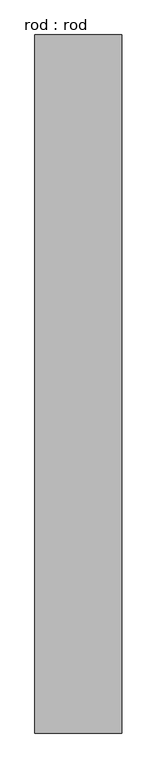
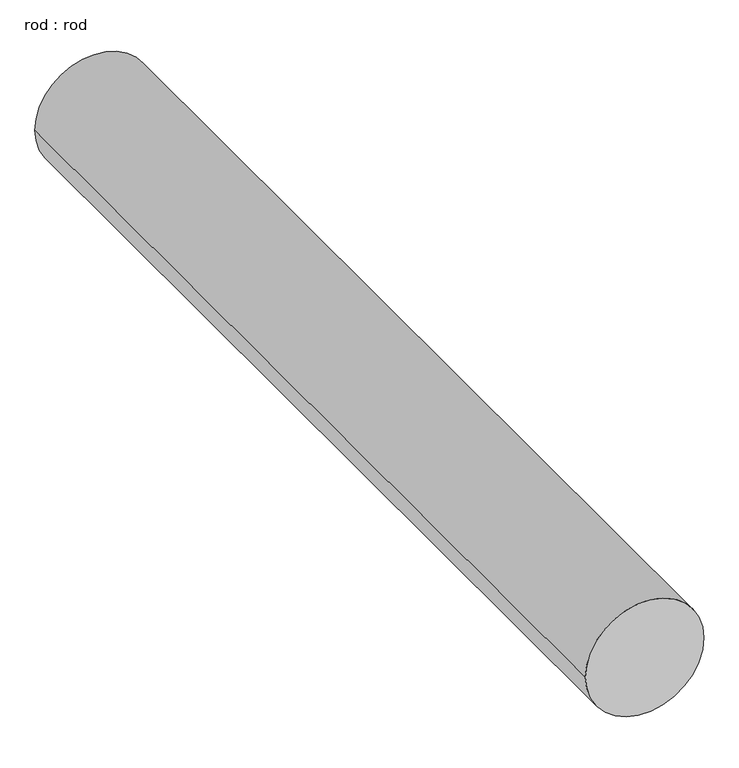
"""IFC4 building model written with IfcOpenShell, lengths in millimetres: proxy geometry, rod : rod."""

from ifc_helpers import new_model, si_unit, point, frame, frame_2d, origin, place, context, project, spatial, circle_curve, trimmed, segment, composite_curve, outline, extrude, source, transform, mapped, element, save


def rod_rod_560d6ef0(model_context):
    return source(origin(), model_context, "Body", "SweptSolid", [
        extrude(outline(composite_curve([segment(trimmed(circle_curve(frame_2d((0.0108462, 0.0)), 200.0), [point((0.0108462, 200.0))], [point((0.0108462, -200.0))], False, "CARTESIAN"), True, "CONTINUOUS"), segment(trimmed(circle_curve(frame_2d((0.0108462, 0.0)), 200.0), [point((0.0108462, -200.0))], [point((0.0108462, 200.0))], False, "CARTESIAN"), True, "CONTINUOUS")], self_intersect=False)), frame((0.0, 2482.7286153, 0.0), z_axis=(0.0, 1.0, 0.0), x_axis=(0.0, 0.0, 1.0)), (0.0, 0.0, 1.0), 3220.0),
    ])


if __name__ == "__main__":
    model = new_model("IFC4")
    model_context = context("Model", 3, world=origin())
    ifc_project = project(units=[si_unit("LENGTHUNIT", "METRE", prefix="MILLI")], contexts=[model_context])
    site = spatial("IfcSite", under=ifc_project)
    building = spatial("IfcBuilding", under=site)
    placement = place(None, origin())
    rod_rod_shape = rod_rod_560d6ef0(model_context)
    element("IfcBuildingElementProxy", 1, Name="rod : rod", ObjectType="rod : rod", at=placement, inside=building, context=model_context, shape_type="MappedRepresentation", body=[
        mapped(rod_rod_shape, transform((0.0, 0.0, 0.0), x_axis=(1.0, 0.0, 0.0), y_axis=(0.0, 1.0, 0.0), z_axis=(0.0, 0.0, 1.0))),
    ])
    save(model, "model.ifc")

# Revit data of these elements
# Type "rod : rod"
#   Default Elevation = 0
